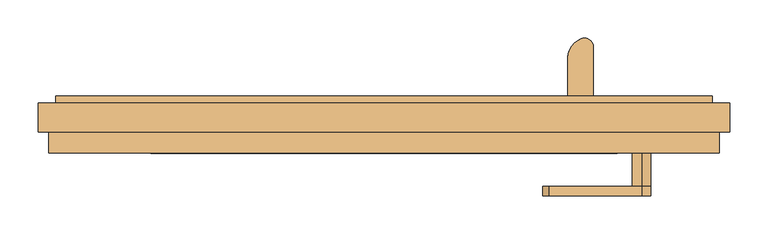
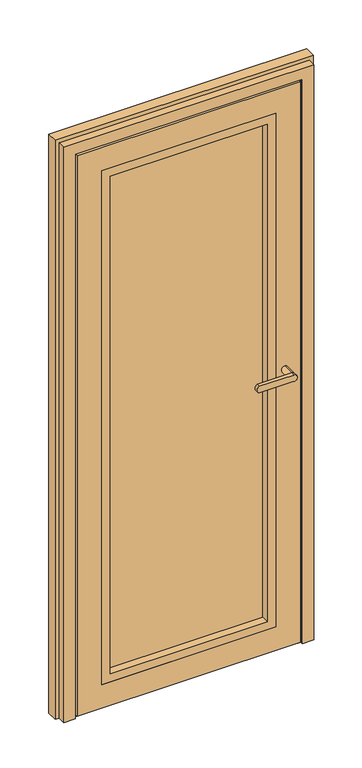
"""IFC4 building model written with IfcOpenShell, lengths in millimetres: door geometry, Schueco_FWS_ADS-75-SimplySmart_inw_Family-01 : FWS SI insert unit."""

from ifc_helpers import new_model, si_unit, point, frame, frame_2d, origin, place, context, project, spatial, polyline, circle_curve, ellipse_curve, trimmed, segment, composite_curve, outline, extrude, faceted_brep, source, transform, mapped, element, save
from ifc_brep_helpers import plane_surface, cylinder_surface, extruded_surface, advanced_brep


def door_e8eff683(model_context):
    return source(origin(), model_context, "Body", "SolidModel", [
        extrude(outline(composite_curve([segment(polyline([(241.3326764, 8.9997177), (241.3326764, 59.1618682)]), True, "CONTINUOUS"), segment(trimmed(circle_curve(frame_2d((268.5110941, 59.1618682)), 27.1784177), [point((241.3326764, 59.1618682))], [point((258.9739985, 84.6120194))], False, "CARTESIAN"), True, "CONTINUOUS"), segment(trimmed(circle_curve(frame_2d((263.0514995, 73.7310321)), 11.6198924), [point((258.9739985, 84.6120194))], [point((274.6713919, 73.7310321))], False, "CARTESIAN"), True, "CONTINUOUS"), segment(polyline([(274.6713919, 73.7310321), (274.6713919, 8.9997177), (241.3326764, 8.9997177)]), True, "CONTINUOUS")], self_intersect=False)), frame((0.0, 0.0, 2046.9218203), z_axis=(0.0, 0.0, 1.0), x_axis=(1.0, 0.0, 0.0)), (0.0, 0.0, 1.0), 4.0),
        extrude(outline(polyline([(241.3326764, 12.9997177), (274.6713919, 12.9997177), (274.6713919, 8.9997177), (241.3326764, 8.9997177), (241.3326764, 12.9997177)])), frame((0.0, 0.0, 2016.9218203), z_axis=(0.0, 0.0, 1.0), x_axis=(1.0, 0.0, 0.0)), (0.0, 0.0, 1.0), 30.0),
        extrude(outline(polyline([(241.3326764, 12.9997177), (274.6713919, 12.9997177), (274.6713919, 8.9997177), (241.3326764, 8.9997177), (241.3326764, 12.9997177)])), frame((0.0, 0.0, 49.9218203), z_axis=(0.0, 0.0, 1.0), x_axis=(1.0, 0.0, 0.0)), (0.0, 0.0, 1.0), 30.0),
        extrude(outline(composite_curve([segment(polyline([(241.3326764, 8.9997177), (241.3326764, 59.1618682)]), True, "CONTINUOUS"), segment(trimmed(circle_curve(frame_2d((268.5110941, 59.1618682)), 27.1784177), [point((241.3326764, 59.1618682))], [point((258.9739985, 84.6120194))], False, "CARTESIAN"), True, "CONTINUOUS"), segment(trimmed(circle_curve(frame_2d((263.0514995, 73.7310321)), 11.6198924), [point((258.9739985, 84.6120194))], [point((274.6713919, 73.7310321))], False, "CARTESIAN"), True, "CONTINUOUS"), segment(polyline([(274.6713919, 73.7310321), (274.6713919, 8.9997177), (241.3326764, 8.9997177)]), True, "CONTINUOUS")], self_intersect=False)), frame((0.0, 0.0, 45.9218203), z_axis=(0.0, 0.0, 1.0), x_axis=(1.0, 0.0, 0.0)), (0.0, 0.0, 1.0), 4.0),
        advanced_brep(
        [(270.717076, 57.5977179, 2046.9218203), (245.282924, 72.2821425, 2046.9218203), (270.717076, 57.5977179, 49.9218203), (245.282924, 72.2821425, 49.9218203)],
        [
            (0, 1, ellipse_curve(frame((258.0, 64.9399302, 2046.9218203), z_axis=(0.0, 0.0, 1.0000000000000002), x_axis=(0.5000002582658958, 0.866025254674503, 0.0)), 21.5840887, 14.6844171)),
            (1, 0, ellipse_curve(frame((258.0, 64.9399302, 2046.9218203), z_axis=(0.0, 0.0, 1.0000000000000002), x_axis=(0.5000002582658958, 0.866025254674503, 0.0)), 21.5840887, 14.6844171)),
            (2, 3, ellipse_curve(frame((258.0, 64.9399302, 49.9218203), z_axis=(0.0, 0.0, -1.0000000000000002), x_axis=(-0.866025254674503, 0.5000002582658958, 0.0)), 14.6844171, 21.5840887)),
            (3, 2, ellipse_curve(frame((258.0, 64.9399302, 49.9218203), z_axis=(0.0, 0.0, -1.0000000000000002), x_axis=(-0.866025254674503, 0.5000002582658958, 0.0)), 14.6844171, 21.5840887)),
            (0, 2),
            (3, 1),
        ],
        [
            plane_surface(frame((245.282924, 72.2821425, 2046.9218203), z_axis=(0.0, 0.0, 1.0000000000000002), x_axis=(0.5000002582658958, 0.866025254674503, 0.0))),
            plane_surface(frame((245.282924, 72.2821425, 49.9218203), z_axis=(0.0, 0.0, -1.0000000000000002), x_axis=(-0.5000002582658958, -0.866025254674503, 0.0))),
            extruded_surface(trimmed(ellipse_curve(frame((258.0, 64.9399302, 49.9218203), z_axis=(0.0, 0.0, -1.0000000000000002), x_axis=(-0.866025254674503, 0.5000002582658958, 0.0)), 14.6844171, 21.5840887), [point((245.282924, 72.2821425, 49.9218203))], [point((270.717076, 57.5977179, 49.9218203))], True, "CARTESIAN"), (0.0, 0.0, -1997.0), 1997.0),
            extruded_surface(trimmed(ellipse_curve(frame((258.0, 64.9399302, 49.9218203), z_axis=(0.0, 0.0, -1.0000000000000002), x_axis=(-0.866025254674503, 0.5000002582658958, 0.0)), 14.6844171, 21.5840887), [point((270.717076, 57.5977179, 49.9218203))], [point((245.282924, 72.2821425, 49.9218203))], True, "CARTESIAN"), (0.0, 0.0, -1997.0), 1997.0),
        ],
        [
            (0, [[1, 2]]),
            (1, [[3, 4]]),
            (2, [[5, -4, 6, -1]]),
            (3, [[-6, -3, -5, -2]]),
        ],
    ),
        advanced_brep(
        [(338.0, -122.0002518, 1030.9991882), (338.0, -122.0002518, 1054.9764498), (216.3382074, -122.0002518, 1054.9764498), (216.3382074, -122.0002518, 1030.9991882), (338.0, -109.5001648, 1054.9764498), (338.0, -109.5001648, 1030.9991882), (216.3382074, -109.5001648, 1030.9991882), (216.3382074, -109.5001648, 1054.9764498), (338.0, -66.0002823, 1030.9991882), (338.0, -66.0002823, 1054.9764498)],
        [
            (0, 1, circle_curve(frame((338.0, -122.0002518, 1042.987819), z_axis=(0.0, -1.0, 0.0), x_axis=(0.0, 0.0, 1.0)), 11.9886308)),
            (1, 2),
            (2, 3, ellipse_curve(frame((216.3382074, -122.0002518, 1042.987819), z_axis=(0.0, -1.0, 0.0), x_axis=(0.0, 0.0, -1.0)), 11.9886308, 7.9050795)),
            (3, 0),
            (4, 5, circle_curve(frame((338.0, -109.5001648, 1042.987819), z_axis=(0.0, -1.0, 0.0), x_axis=(0.0, 0.0, 1.0)), 11.9886308)),
            (5, 6),
            (6, 7, ellipse_curve(frame((216.3382074, -109.5001648, 1042.987819), z_axis=(0.0, 1.0, 0.0), x_axis=(0.0, 0.0, -1.0)), 11.9886308, 7.9050795)),
            (7, 4),
            (3, 6),
            (5, 0),
            (2, 7),
            (1, 4),
            (5, 4, circle_curve(frame((338.0, -109.5001648, 1042.987819), z_axis=(0.0, -1.0, 0.0), x_axis=(0.0, 0.0, 1.0)), 11.9886308)),
            (8, 9, circle_curve(frame((338.0, -66.0002823, 1042.987819), z_axis=(0.0, 1.0, 0.0), x_axis=(0.0, 0.0, 1.0)), 11.9886308)),
            (9, 8, circle_curve(frame((338.0, -66.0002823, 1042.987819), z_axis=(0.0, 1.0, 0.0), x_axis=(0.0, 0.0, 1.0)), 11.9886308)),
            (8, 5),
            (4, 9),
        ],
        [
            plane_surface(frame((216.3382074, -122.0002518, 1030.9991882), z_axis=(0.0, -1.0, 0.0), x_axis=(-1.0, 0.0, 0.0))),
            plane_surface(frame((216.3382074, -109.5001648, 1030.9991882), z_axis=(0.0, 1.0, 0.0), x_axis=(1.0, 0.0, 0.0))),
            plane_surface(frame((338.0, -122.0002518, 1030.9991882), z_axis=(0.0, 0.0, -1.0), x_axis=(0.0, 1.0, 0.0))),
            extruded_surface(trimmed(ellipse_curve(frame((216.3382074, -109.5001648, 1042.987819), z_axis=(0.0, 1.0, 0.0), x_axis=(0.0, 0.0, -1.0)), 11.9886308, 7.9050795), [point((216.3382074, -109.5001648, 1030.9991882))], [point((216.3382074, -109.5001648, 1054.9764498))], True, "CARTESIAN"), (0.0, 12.500086999999994, 0.0), 12.500086999999994),
            plane_surface(frame((216.3382074, -122.0002518, 1054.9764498), z_axis=(0.0, 0.0, 1.0), x_axis=(0.0, 1.0, 0.0))),
            cylinder_surface(frame((338.0, -109.5001648, 1042.987819), z_axis=(0.0, -1.0, 0.0), x_axis=(0.0, 0.0, 1.0)), 11.9886308),
            plane_surface(frame((338.0, -66.0002823, 1054.9764498), z_axis=(0.0, 1.0, 0.0), x_axis=(-1.0, 0.0, 0.0))),
            cylinder_surface(frame((338.0, -66.0002823, 1042.987819), z_axis=(0.0, -1.0, 0.0), x_axis=(0.0, 0.0, 1.0)), 11.9886308),
        ],
        [
            (0, [[1, 2, 3, 4]]),
            (1, [[5, 6, 7, 8]]),
            (2, [[9, -6, 10, -4]]),
            (3, [[11, -7, -9, -3]]),
            (4, [[12, -8, -11, -2]]),
            (5, [[-10, 13, -12, -1]]),
            (6, [[14, 15]]),
            (7, [[16, -5, 17, -14]]),
            (7, [[-17, -13, -16, -15]]),
        ],
    ),
        extrude(outline(polyline([(94.987819, 306.0), (2005.987819, 306.0), (2005.987819, -306.0), (94.987819, -306.0), (94.987819, 306.0)]), holes=[polyline([(124.987819, -276.0), (1975.987819, -276.0), (1975.987819, 276.0), (124.987819, 276.0), (124.987819, -276.0)])]), frame((0.0, -66.0002823, 0.0), z_axis=(0.0, 1.0, 0.0), x_axis=(0.0, 0.0, 1.0)), (0.0, 0.0, 1.0), 28.0002823),
        faceted_brep([(-393.0, -66.0002823, 2092.987819), (-393.0, -57.5000065, 2092.987819), (-393.0, -57.5000065, 7.987819), (-393.0, -66.0002823, 7.987819), (393.0, -57.5000065, 7.987819), (393.0, -66.0002823, 7.987819), (393.0, -57.5000065, 2092.987819), (374.0, -57.5000065, 26.987819), (374.0, -57.5000065, 2073.987819), (-374.0, -57.5000065, 2073.987819), (-374.0, -57.5000065, 26.987819), (393.0, -66.0002823, 2092.987819), (-306.0, -66.0002823, 94.987819), (-306.0, -66.0002823, 2005.987819), (306.0, -66.0002823, 2005.987819), (306.0, -66.0002823, 94.987819), (-306.0, 0.0, 2005.987819), (-306.0, 0.0, 94.987819), (306.0, 0.0, 94.987819), (306.0, 0.0, 2005.987819), (-274.0, 0.0, 126.987819), (-274.0, 0.0, 1973.987819), (274.0, 0.0, 1973.987819), (274.0, 0.0, 126.987819), (-274.0, 8.9997177, 1973.987819), (-274.0, 8.9997177, 126.987819), (274.0, 8.9997177, 126.987819), (274.0, 8.9997177, 1973.987819), (-361.0, 8.9997177, 39.987819), (-361.0, 8.9997177, 2060.987819), (361.0, 8.9997177, 2060.987819), (361.0, 8.9997177, 39.987819), (-361.0, 0.4997603, 2060.987819), (-361.0, 0.4997603, 39.987819), (361.0, 0.4997603, 39.987819), (361.0, 0.4997603, 2060.987819), (-374.0, 0.4997603, 26.987819), (-374.0, 0.4997603, 2073.987819), (374.0, 0.4997603, 2073.987819), (374.0, 0.4997603, 26.987819)], [[[0, 1, 2, 3]], [[3, 2, 4, 5]], [[2, 1, 6, 4], [7, 8, 9, 10]], [[5, 4, 6, 11]], [[5, 11, 0, 3], [12, 13, 14, 15]], [[16, 13, 12, 17]], [[17, 12, 15, 18]], [[18, 15, 14, 19]], [[18, 19, 16, 17], [20, 21, 22, 23]], [[24, 21, 20, 25]], [[25, 20, 23, 26]], [[26, 23, 22, 27]], [[28, 29, 30, 31], [26, 27, 24, 25]], [[32, 29, 28, 33]], [[33, 28, 31, 34]], [[34, 31, 30, 35]], [[36, 37, 38, 39], [34, 35, 32, 33]], [[9, 37, 36, 10]], [[10, 36, 39, 7]], [[7, 39, 38, 8]], [[11, 6, 1, 0]], [[19, 14, 13, 16]], [[27, 22, 21, 24]], [[35, 30, 29, 32]], [[8, 38, 37, 9]]]),
        extrude(outline(polyline([(306.0, -38.0), (-306.0, -38.0), (-306.0, 0.0), (306.0, 0.0), (306.0, -38.0)])), frame((0.0, 0.0, 94.987819), z_axis=(0.0, 0.0, 1.0), x_axis=(1.0, 0.0, 0.0)), (0.0, 0.0, 1.0), 1911.0),
        extrude(outline(composite_curve([segment(polyline([(-39.1486683, 26.987819), (-17.8439358, 26.987819), (-17.8439358, 3.5881205)]), True, "CONTINUOUS"), segment(trimmed(circle_curve(frame_2d((-28.496302, 19.4783613)), 19.1304119), [point((-17.8439358, 3.5881205))], [point((-39.1486683, 3.5881205))], False, "CARTESIAN"), True, "CONTINUOUS"), segment(polyline([(-39.1486683, 3.5881205), (-39.1486683, 26.987819)]), True, "CONTINUOUS")], self_intersect=False)), frame((-374.0, 0.0, 0.0), z_axis=(1.0, 0.0, 0.0), x_axis=(0.0, 1.0, 0.0)), (0.0, 0.0, 1.0), 748.0),
        extrude(outline(polyline([(-361.0, 0.4997603), (-361.0, 8.9997177), (361.0, 8.9997177), (361.0, 0.4997603), (-361.0, 0.4997603)])), frame((0.0, 0.0, 7.987819), z_axis=(0.0, 0.0, 1.0), x_axis=(1.0, 0.0, 0.0)), (0.0, 0.0, 1.0), 32.0),
        faceted_brep([(430.999943, 8.9997177, 2130.999943), (430.999943, 0.0, 2130.999943), (430.999943, 0.0, 0.0), (430.999943, 8.9997177, 0.0), (-454.0, 0.0, 0.0), (-454.0, 0.0, 2154.0), (454.0, 0.0, 2154.0), (454.0, 0.0, 0.0), (-430.999943, 0.0, 2130.999943), (-430.999943, 0.0, 0.0), (454.0, -38.0, 0.0), (440.0, -38.0, 0.0), (440.0, -66.0002823, 0.0), (399.9999732, -66.0002823, 0.0), (399.9999732, -57.5000065, 0.0), (388.4999732, -57.5000065, 0.0), (388.4999732, 0.4997603, 0.0), (367.9999732, 0.4997603, 0.0), (367.9999732, 8.9997177, 0.0), (-367.9999732, 8.9997177, 0.0), (-430.999943, 8.9997177, 0.0), (-430.999943, 8.9997177, 2130.999943), (367.9999732, 8.9997177, 2067.9999732), (-367.9999732, 8.9997177, 2067.9999732), (399.9999732, -66.0002823, 2099.9999732), (399.9999732, -57.5000065, 2099.9999732), (-399.9999732, -57.5000065, 0.0), (-388.4999732, -57.5000065, 0.0), (-388.4999732, -57.5000065, 2088.4999732), (388.4999732, -57.5000065, 2088.4999732), (-399.9999732, -57.5000065, 2099.9999732), (-440.0, -66.0002823, 0.0), (-399.9999732, -66.0002823, 0.0), (-399.9999732, -66.0002823, 2099.9999732), (440.0, -66.0002823, 2140.0), (-440.0, -66.0002823, 2140.0), (440.0, -38.0, 2140.0), (-454.0, -38.0, 0.0), (-440.0, -38.0, 0.0), (-440.0, -38.0, 2140.0), (454.0, -38.0, 2154.0), (-454.0, -38.0, 2154.0), (-367.9999732, 0.4997603, 0.0), (-388.4999732, 0.4997603, 0.0), (367.9999732, 0.4997603, 2067.9999732), (-367.9999732, 0.4997603, 2067.9999732), (388.4999732, 0.4997603, 2088.4999732), (-388.4999732, 0.4997603, 2088.4999732)], [[[0, 1, 2, 3]], [[4, 5, 6, 7, 2, 1, 8, 9]], [[3, 2, 7, 10, 11, 12, 13, 14, 15, 16, 17, 18]], [[19, 20, 21, 0, 3, 18, 22, 23]], [[24, 25, 14, 13]], [[26, 27, 28, 29, 15, 14, 25, 30]], [[31, 32, 33, 24, 13, 12, 34, 35]], [[34, 12, 11, 36]], [[37, 38, 39, 36, 11, 10, 40, 41]], [[4, 9, 20, 19, 42, 43, 27, 26, 32, 31, 38, 37]], [[20, 9, 8, 21]], [[18, 17, 44, 22]], [[42, 19, 23, 45]], [[32, 26, 30, 33]], [[31, 35, 39, 38]], [[4, 37, 41, 5]], [[6, 40, 10, 7]], [[43, 42, 45, 44, 17, 16, 46, 47]], [[16, 15, 29, 46]], [[27, 43, 47, 28]], [[21, 8, 1, 0]], [[33, 30, 25, 24]], [[35, 34, 36, 39]], [[23, 22, 44, 45]], [[5, 41, 40, 6]], [[47, 46, 29, 28]]]),
    ])


if __name__ == "__main__":
    model = new_model("IFC4")
    model_context = context("Model", 3, world=origin())
    ifc_project = project(units=[si_unit("LENGTHUNIT", "METRE", prefix="MILLI")], contexts=[model_context])
    site = spatial("IfcSite", under=ifc_project)
    building = spatial("IfcBuilding", under=site)
    placement = place(None, origin())
    door_shape = door_e8eff683(model_context)
    element("IfcDoor", 1, ObjectType="Schueco_FWS_ADS-75-SimplySmart_inw_Family-01 : FWS SI insert unit", at=placement, inside=building, context=model_context, shape_type="MappedRepresentation", body=[
        mapped(door_shape, transform((0.0, 0.0, 0.0), x_axis=(1.0, 0.0, 0.0), y_axis=(0.0, 1.0, 0.0), z_axis=(0.0, 0.0, 1.0))),
    ])
    save(model, "model.ifc")

# Revit data of these elements
# Type "Schueco_FWS_ADS-75-SimplySmart_inw_Family-01 : FWS SI insert unit"
#   Type Mark = "53"
#   __NOTE__ = "Data describes the optimum values of the entire system. The properites of a selected design option have to be determined on an individual basis!"
#   Wind load resistance = "Class C3"
#   Watertightness = "Class E750"
#   Thermal insulation = "Uf = 1.6 W/(m²K)"
#   Sound insulation = "..."
#   Schueco thermal insulation standard = "Highly thermally insulated"
#   Opening type = "Inward-opening, Flush-fitted"
#   Model = "Schueco ADS 75 SimplySmart"
#   Mechanical loading = "..."
#   Maximum leaf width in mm = "1400"
#   Maximum leaf weight in kg = "200"
#   Maximum leaf height in mm = "3000"
#   Material = "Aluminium"
#   Construction Type = "Door, single-leaf, inward-opening"
#   Manufacturer = "Schueco International KG"
#   Long term functionality = "..."
#   Glazing data = "Triple glazing 38mm"
#   Façade insert unit = "yes"
#   Family creation date = "08.2017"
#   Description = "Schueco Aluminium Door System (ADS)"
#   Burglar resistance = "Class RC 2"
#   Areas of use = "Public buildings, Residential buildings, Side entrance"
#   Analytic Construction = "<None>"
#   Air permeability = "Class 4"
#   Width [instance default] = 946.941 mm
#   Leaf opening angle [instance default] = 0.00°
#   IOf_T = 38 mm
#   Height [instance default] = 1988.68 mm
#   Glazing area [instance default] = 0.987046 m²
#   Distance from bottom to handles [instance default] = 1050 mm
#   Clear opening width [instance default] = 774.941 mm
#   Standard threshold = no
#   Low level threshold = yes
#   Handles = yes
#   Glass = none
#   Frame = Alu
#   Fittings = none
# Element 1 (IfcDoor, "Schueco_FWS_ADS-75-SimplySmart_inw_Family-01 : FWS SI insert unit")
#   Width = 908 mm
#   Height = 2154 mm
#   Glazing area = 1.01216 m²
#   Clear opening width = 736 mm
#   Materials on its faces: "Alu", "Glass"
# Materials
#   "Alu": class "Glas", colour RGB 140 140 140, transparency 0
#   "Glass": class "Glass", colour RGB 128 128 255, transparency 0.75, Description = "Soda Lime Glass", Cost = 0
